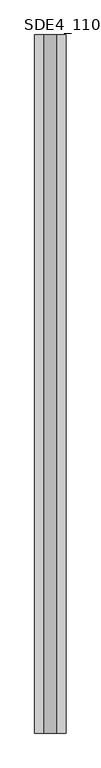
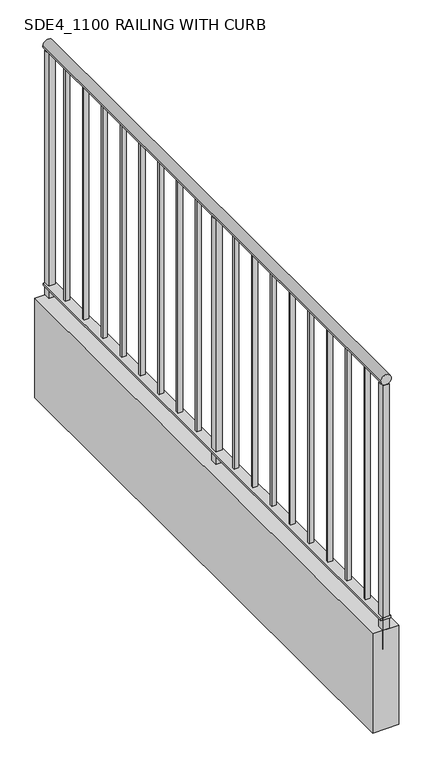
"""IFC4 building model written with IfcOpenShell, lengths in millimetres: railing geometry, SDE4_1100 RAILING WITH CURB."""

from ifc_helpers import new_model, si_unit, point, frame, frame_2d, origin, place, context, project, spatial, polyline, circle_curve, trimmed, segment, composite_curve, outline, extrude, source, transform, mapped, element, save


def sde4_1100_railing_with_curb_933cecba(model_context):
    return source(origin(), model_context, "Body", "SweptSolid", [
        extrude(outline(composite_curve([segment(trimmed(circle_curve(frame_2d((131550.0, 76500.4)), 20.0), [point((131550.0, 76520.4))], [point((131550.0, 76480.4))], False, "CARTESIAN"), True, "CONTINUOUS"), segment(trimmed(circle_curve(frame_2d((131550.0, 76500.4)), 20.0), [point((131550.0, 76480.4))], [point((131550.0, 76520.4))], False, "CARTESIAN"), True, "CONTINUOUS")], self_intersect=False)), frame((0.0, 11427.5856435, 0.0), z_axis=(0.0, 1.0, 0.0), x_axis=(0.0, 0.0, 1.0)), (0.0, 0.0, 1.0), 2227.9721935),
        extrude(outline(polyline([(76481.4, 13655.557837), (76519.4, 13655.557837), (76519.4, 11427.5856435), (76481.4, 11427.5856435), (76481.4, 13655.557837)])), frame((0.0, 0.0, 130586.0), z_axis=(0.0, 0.0, 1.0), x_axis=(1.0, 0.0, 0.0)), (0.0, 0.0, 1.0), 9.0),
        extrude(outline(polyline([(76450.0, 13655.557837), (76550.0, 13655.557837), (76550.0, 11427.5856435), (76450.0, 11427.5856435), (76450.0, 13655.557837)])), frame((0.0, 0.0, 130145.0), z_axis=(0.0, 0.0, 1.0), x_axis=(1.0, 0.0, 0.0)), (0.0, 0.0, 1.0), 400.0),
        extrude(outline(polyline([(76491.4, 11555.8618765), (76509.4, 11555.8618765), (76509.4, 11546.8618765), (76491.4, 11546.8618765), (76491.4, 11555.8618765)])), frame((0.0, 0.0, 130595.0), z_axis=(0.0, 0.0, 1.0), x_axis=(1.0, 0.0, 0.0)), (0.0, 0.0, 1.0), 935.0),
        extrude(outline(polyline([(76491.4, 11679.6381095), (76509.4, 11679.6381095), (76509.4, 11670.6381095), (76491.4, 11670.6381095), (76491.4, 11679.6381095)])), frame((0.0, 0.0, 130595.0), z_axis=(0.0, 0.0, 1.0), x_axis=(1.0, 0.0, 0.0)), (0.0, 0.0, 1.0), 935.0),
        extrude(outline(polyline([(76491.4, 11803.4143425), (76509.4, 11803.4143425), (76509.4, 11794.4143425), (76491.4, 11794.4143425), (76491.4, 11803.4143425)])), frame((0.0, 0.0, 130595.0), z_axis=(0.0, 0.0, 1.0), x_axis=(1.0, 0.0, 0.0)), (0.0, 0.0, 1.0), 935.0),
        extrude(outline(polyline([(76491.4, 11927.1905754), (76509.4, 11927.1905754), (76509.4, 11918.1905754), (76491.4, 11918.1905754), (76491.4, 11927.1905754)])), frame((0.0, 0.0, 130595.0), z_axis=(0.0, 0.0, 1.0), x_axis=(1.0, 0.0, 0.0)), (0.0, 0.0, 1.0), 935.0),
        extrude(outline(polyline([(76491.4, 12050.9668084), (76509.4, 12050.9668084), (76509.4, 12041.9668084), (76491.4, 12041.9668084), (76491.4, 12050.9668084)])), frame((0.0, 0.0, 130595.0), z_axis=(0.0, 0.0, 1.0), x_axis=(1.0, 0.0, 0.0)), (0.0, 0.0, 1.0), 935.0),
        extrude(outline(polyline([(76491.4, 12174.7430414), (76509.4, 12174.7430414), (76509.4, 12165.7430414), (76491.4, 12165.7430414), (76491.4, 12174.7430414)])), frame((0.0, 0.0, 130595.0), z_axis=(0.0, 0.0, 1.0), x_axis=(1.0, 0.0, 0.0)), (0.0, 0.0, 1.0), 935.0),
        extrude(outline(polyline([(76491.4, 12298.5192744), (76509.4, 12298.5192744), (76509.4, 12289.5192744), (76491.4, 12289.5192744), (76491.4, 12298.5192744)])), frame((0.0, 0.0, 130595.0), z_axis=(0.0, 0.0, 1.0), x_axis=(1.0, 0.0, 0.0)), (0.0, 0.0, 1.0), 935.0),
        extrude(outline(polyline([(76491.4, 12422.2955073), (76509.4, 12422.2955073), (76509.4, 12413.2955073), (76491.4, 12413.2955073), (76491.4, 12422.2955073)])), frame((0.0, 0.0, 130595.0), z_axis=(0.0, 0.0, 1.0), x_axis=(1.0, 0.0, 0.0)), (0.0, 0.0, 1.0), 935.0),
        extrude(outline(polyline([(76487.9, 12554.0717403), (76512.9, 12554.0717403), (76512.9, 12529.0717403), (76487.9, 12529.0717403), (76487.9, 12554.0717403)])), frame((0.0, 0.0, 130545.0), z_axis=(0.0, 0.0, 1.0), x_axis=(1.0, 0.0, 0.0)), (0.0, 0.0, 1.0), 985.0),
        extrude(outline(polyline([(76491.4, 12669.8479733), (76509.4, 12669.8479733), (76509.4, 12660.8479733), (76491.4, 12660.8479733), (76491.4, 12669.8479733)])), frame((0.0, 0.0, 130595.0), z_axis=(0.0, 0.0, 1.0), x_axis=(1.0, 0.0, 0.0)), (0.0, 0.0, 1.0), 935.0),
        extrude(outline(polyline([(76491.4, 12793.6242062), (76509.4, 12793.6242062), (76509.4, 12784.6242062), (76491.4, 12784.6242062), (76491.4, 12793.6242062)])), frame((0.0, 0.0, 130595.0), z_axis=(0.0, 0.0, 1.0), x_axis=(1.0, 0.0, 0.0)), (0.0, 0.0, 1.0), 935.0),
        extrude(outline(polyline([(76491.4, 12917.4004392), (76509.4, 12917.4004392), (76509.4, 12908.4004392), (76491.4, 12908.4004392), (76491.4, 12917.4004392)])), frame((0.0, 0.0, 130595.0), z_axis=(0.0, 0.0, 1.0), x_axis=(1.0, 0.0, 0.0)), (0.0, 0.0, 1.0), 935.0),
        extrude(outline(polyline([(76491.4, 13041.1766722), (76509.4, 13041.1766722), (76509.4, 13032.1766722), (76491.4, 13032.1766722), (76491.4, 13041.1766722)])), frame((0.0, 0.0, 130595.0), z_axis=(0.0, 0.0, 1.0), x_axis=(1.0, 0.0, 0.0)), (0.0, 0.0, 1.0), 935.0),
        extrude(outline(polyline([(76491.4, 13164.9529052), (76509.4, 13164.9529052), (76509.4, 13155.9529052), (76491.4, 13155.9529052), (76491.4, 13164.9529052)])), frame((0.0, 0.0, 130595.0), z_axis=(0.0, 0.0, 1.0), x_axis=(1.0, 0.0, 0.0)), (0.0, 0.0, 1.0), 935.0),
        extrude(outline(polyline([(76491.4, 13288.7291381), (76509.4, 13288.7291381), (76509.4, 13279.7291381), (76491.4, 13279.7291381), (76491.4, 13288.7291381)])), frame((0.0, 0.0, 130595.0), z_axis=(0.0, 0.0, 1.0), x_axis=(1.0, 0.0, 0.0)), (0.0, 0.0, 1.0), 935.0),
        extrude(outline(polyline([(76491.4, 13412.5053711), (76509.4, 13412.5053711), (76509.4, 13403.5053711), (76491.4, 13403.5053711), (76491.4, 13412.5053711)])), frame((0.0, 0.0, 130595.0), z_axis=(0.0, 0.0, 1.0), x_axis=(1.0, 0.0, 0.0)), (0.0, 0.0, 1.0), 935.0),
        extrude(outline(polyline([(76491.4, 13536.2816041), (76509.4, 13536.2816041), (76509.4, 13527.2816041), (76491.4, 13527.2816041), (76491.4, 13536.2816041)])), frame((0.0, 0.0, 130595.0), z_axis=(0.0, 0.0, 1.0), x_axis=(1.0, 0.0, 0.0)), (0.0, 0.0, 1.0), 935.0),
        extrude(outline(polyline([(76512.9, 11452.5856435), (76512.9, 11427.5856435), (76487.9, 11427.5856435), (76487.9, 11452.5856435), (76512.9, 11452.5856435)])), frame((0.0, 0.0, 130470.0), z_axis=(0.0, 0.0, 1.0), x_axis=(1.0, 0.0, 0.0)), (0.0, 0.0, 1.0), 1060.0),
        extrude(outline(polyline([(76512.9, 13655.557837), (76512.9, 13630.557837), (76487.9, 13630.557837), (76487.9, 13655.557837), (76512.9, 13655.557837)])), frame((0.0, 0.0, 130470.0), z_axis=(0.0, 0.0, 1.0), x_axis=(1.0, 0.0, 0.0)), (0.0, 0.0, 1.0), 1060.0),
    ])


if __name__ == "__main__":
    model = new_model("IFC4")
    model_context = context("Model", 3, world=origin())
    ifc_project = project(units=[si_unit("LENGTHUNIT", "METRE", prefix="MILLI")], contexts=[model_context])
    site = spatial("IfcSite", under=ifc_project)
    building = spatial("IfcBuilding", under=site)
    placement = place(None, origin())
    sde4_1100_railing_with_curb_shape = sde4_1100_railing_with_curb_933cecba(model_context)
    element("IfcRailing", 1, ObjectType="SDE4_1100 RAILING WITH CURB", at=placement, inside=building, context=model_context, shape_type="MappedRepresentation", body=[
        mapped(sde4_1100_railing_with_curb_shape, transform((0.0, 0.0, 0.0), x_axis=(1.0, 0.0, 0.0), y_axis=(0.0, 1.0, 0.0), z_axis=(0.0, 0.0, 1.0))),
    ])
    save(model, "model.ifc")

# Revit data of these elements
# Element 1 (IfcRailing, "SDE4_1100 RAILING WITH CURB")
#   Materials on its faces: "Metal - Steel", "Concrete - Cast-in-Place Concrete"
# Materials
#   "Metal - Steel": class "Metal", colour RGB 247 247 247, transparency 0
#   "Concrete - Cast-in-Place Concrete": class "Concrete", colour RGB 191 178 173, transparency 0, Keynote = "E10/132", Cost = 0
